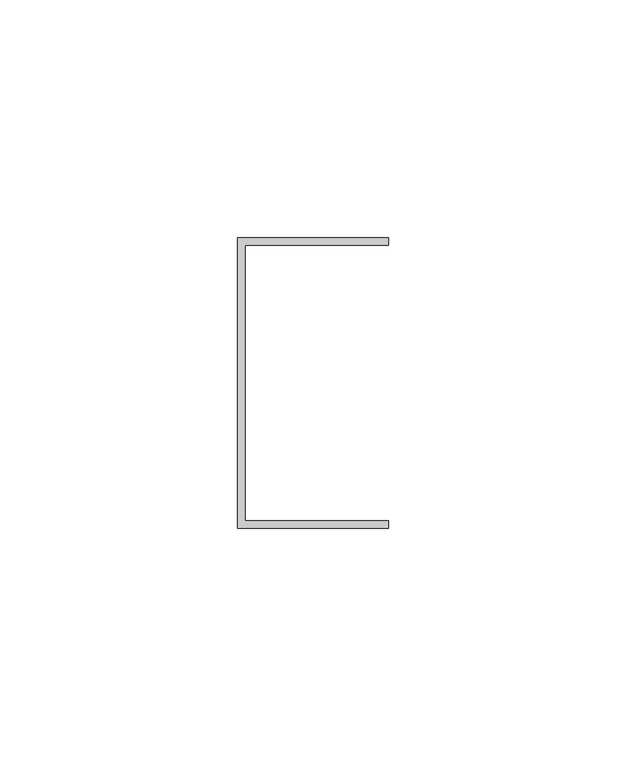
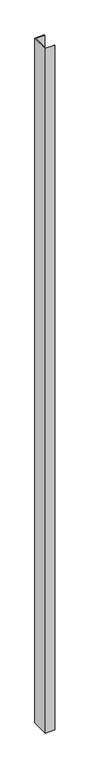
"""IFC4 building model written with IfcOpenShell, lengths in millimetres: proxy geometry, Generic Models 7:Generic Models 1:3:Generic Models 1:3 : Generic Models 7:Generic Models 1:305549:3:Generic Models 1:3:Generic Models 1:3 : Generic Models 7:Generic Models 1:305549:3 : Generic Models 7:Generic Models 1:3:Generic Models 1:3 : Generic Models 7:Generic Models 1:305549:301244:52 : Generic Models 7:Generic Models 1:3:Generic Models 1:3 : Generic Models 7:Generic Models 1:305549:3:Generic Models 1:3:Generic Models 1:3 : Generic Models 7:Generic Models 1:305549:3 : Generic Models 7:Generic Models 1:3:Generic Models 1:3 : Generic Models 7:Generic Models 1:305549:301244:308848."""

from ifc_helpers import new_model, si_unit, frame, origin, place, context, project, spatial, polyline, outline, extrude, source, transform, mapped, element, save


def generic_models_b372dce8(model_context):
    return source(origin(), model_context, "Body", "SweptSolid", [
        extrude(outline(polyline([(578987.0367239, -579015.772634), (579018.7867239, -579015.772634), (579018.7867239, -579017.360134), (578988.6242239, -579017.360134), (578988.6242239, -579075.303884), (579018.7867239, -579075.303884), (579018.7867239, -579076.891384), (578987.0367239, -579076.891384), (578987.0367239, -579015.772634)])), frame((0.0, 0.0, 3721.1), z_axis=(0.0, 0.0, 1.0), x_axis=(1.0, 0.0, 0.0)), (0.0, 0.0, 1.0), 2430.9324376),
    ])


if __name__ == "__main__":
    model = new_model("IFC4")
    model_context = context("Model", 3, world=origin())
    ifc_project = project(units=[si_unit("LENGTHUNIT", "METRE", prefix="MILLI")], contexts=[model_context])
    site = spatial("IfcSite", under=ifc_project)
    building = spatial("IfcBuilding", under=site)
    placement = place(None, origin())
    generic_models_shape = generic_models_b372dce8(model_context)
    element("IfcBuildingElementProxy", 1, Name="Generic Models 7:Generic Models 1:3:Generic Models 1:3 : Generic Models 7:Generic Models 1:305549:3:Generic Models 1:3:Generic Models 1:3 : Generic Models 7:Generic Models 1:305549:3 : Generic Models 7:Generic Models 1:3:Generic Models 1:3 : Generic Models 7:Generic Models 1:305549:301244:52 : Generic Models 7:Generic Models 1:3:Generic Models 1:3 : Generic Models 7:Generic Models 1:305549:3:Generic Models 1:3:Generic Models 1:3 : Generic Models 7:Generic Models 1:305549:3 : Generic Models 7:Generic Models 1:3:Generic Models 1:3 : Generic Models 7:Generic Models 1:305549:301244:308848", ObjectType="Generic Models 7:Generic Models 1:3:Generic Models 1:3 : Generic Models 7:Generic Models 1:305549:3:Generic Models 1:3:Generic Models 1:3 : Generic Models 7:Generic Models 1:305549:3 : Generic Models 7:Generic Models 1:3:Generic Models 1:3 : Generic Models 7:Generic Models 1:305549:301244:52 : Generic Models 7:Generic Models 1:3:Generic Models 1:3 : Generic Models 7:Generic Models 1:305549:3:Generic Models 1:3:Generic Models 1:3 : Generic Models 7:Generic Models 1:305549:3 : Generic Models 7:Generic Models 1:3:Generic Models 1:3 : Generic Models 7:Generic Models 1:305549:301244:308848", at=placement, inside=building, context=model_context, shape_type="MappedRepresentation", body=[
        mapped(generic_models_shape, transform((0.0, 0.0, 0.0), x_axis=(1.0, 0.0, 0.0), y_axis=(0.0, 1.0, 0.0), z_axis=(0.0, 0.0, 1.0))),
    ])
    save(model, "model.ifc")

# Revit data of these elements
# Type "Generic Models 7:Generic Models 1:3:Generic Models 1:3 : Generic Models 7:Generic Models 1:305549:3:Generic Models 1:3:Generic Models 1:3 : Generic Models 7:Generic Models 1:305549:3 : Generic Models 7:Generic Models 1:3:Generic Models 1:3 : Generic Models 7:Generic Models 1:305549:301244:52 : Generic Models 7:Generic Models 1:3:Generic Models 1:3 : Generic Models 7:Generic Models 1:305549:3:Generic Models 1:3:Generic Models 1:3 : Generic Models 7:Generic Models 1:305549:3 : Generic Models 7:Generic Models 1:3:Generic Models 1:3 : Generic Models 7:Generic Models 1:305549:301244:308848"
#   NameOverride = "Generic Models 7:Generic Models 1:3:Generic Models 1:3 : Generic Models 7:Generic Models 1:305549:3:Generic Models 1:3:Generic Models 1:3 : Generic Models 7:Generic Models 1:305549:3 : Generic Models 7:Generic Models 1:3:Generic Models 1:3 : Generic Models 7:Generic Models 1:305549:301244:308848"
#   ObjectTypeOverride = "Generic Models 1:3:Generic Models 1:3 : Generic Models 7:Generic Models 1:305549:3 : Generic Models 7:Generic Models 1:3:Generic Models 1:3 : Generic Models 7:Generic Models 1:305549:301244"
#   Reference = "Generic Models 1"
#   Tag = "308848"
# Element 1 (IfcBuildingElementProxy, "Generic Models 7:Generic Models 1:3:Generic Models 1:3 : Generic Models 7:Generic Models 1:305549:3:Generic Models 1:3:Generic Models 1:3 : Generic Models 7:Generic Models 1:305549:3 : Generic Models 7:Generic Models 1:3:Generic Models 1:3 : Generic Models 7:Generic Models 1:305549:301244:52 : Generic Models 7:Generic Models 1:3:Generic Models 1:3 : Generic Models 7:Generic Models 1:305549:3:Generic Models 1:3:Generic Models 1:3 : Generic Models 7:Generic Models 1:305549:3 : Generic Models 7:Generic Models 1:3:Generic Models 1:3 : Generic Models 7:Generic Models 1:305549:301244:308848")
#   Materials on its faces: "GALVANIZED U-CHANNEL (250T125-33)"
# Materials
#   "GALVANIZED U-CHANNEL (250T125-33)": class "Unassigned", colour RGB 202 201 200, transparency 0, Keynote = "M05451300.02", Cost = 0
